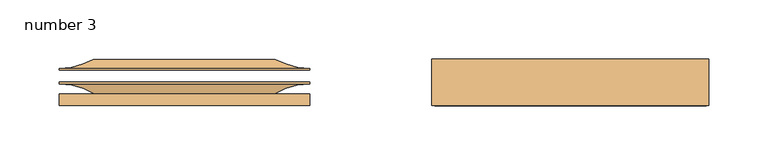
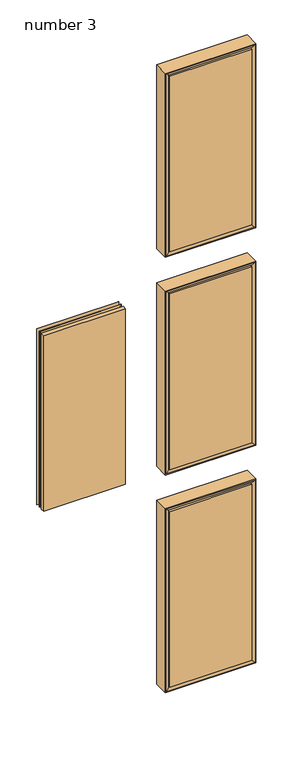
"""IFC4 building model written with IfcOpenShell, lengths in millimetres: door geometry, Door-Interior-Karona-K5660-6_Panel : number 3."""

from ifc_helpers import new_model, si_unit, frame, origin, place, context, project, spatial, polyline, ellipse_curve, source, transform, mapped, element, save
from ifc_brep_helpers import plane_surface, cylinder_surface, revolved_surface, advanced_brep


def number_3_bfdb8d82(model_context):
    return source(origin(), model_context, "Body", "AdvancedBrep", [
        advanced_brep(
        [(268.2748, -54.4576, 1893.8748), (57.1627, -54.4576, 1893.8748), (57.1627, -54.4576, 1414.4752), (268.2748, -54.4576, 1414.4752), (268.2748, -34.7218, 1893.8748), (57.1627, -34.7218, 1893.8748), (57.1627, -36.0454899, 1893.8748), (268.2748, -36.0454899, 1893.8748), (268.2748, -44.5515929, 1893.8748), (57.1627, -44.5515929, 1893.8748), (57.1627, -34.7218, 1414.4752), (268.2748, -34.7218, 1414.4752), (268.2748, -36.0454899, 1414.4752), (57.1627, -36.0454899, 1414.4752), (57.1627, -44.5515929, 1414.4752), (268.2748, -44.5515929, 1414.4752), (87.1686653, -44.5515929, 1863.8688347), (238.2688347, -44.5515929, 1863.8688347), (87.1686653, -44.5515929, 1444.4811653), (238.2688347, -44.5515929, 1444.4811653)],
        [
            (0, 1),
            (1, 2),
            (2, 3),
            (3, 0),
            (4, 5),
            (5, 6),
            (6, 7),
            (7, 4),
            (0, 8),
            (8, 9),
            (9, 1),
            (10, 11),
            (11, 12),
            (12, 13),
            (13, 10),
            (2, 14),
            (14, 15),
            (15, 3),
            (15, 8),
            (11, 4),
            (7, 12),
            (9, 14),
            (5, 10),
            (13, 6),
            (16, 17),
            (17, 7, ellipse_curve(frame((270.2131685, -100.0605261, 1895.8131685), z_axis=(0.7071067811865475, 0.0, -0.7071067811865475), x_axis=(0.7071067811865476, 0.0, 0.7071067811865474)), 90.5724254, 64.0443762)),
            (6, 16, ellipse_curve(frame((55.2243315, -100.0605261, 1895.8131685), z_axis=(-0.7071067811865475, 0.0, -0.7071067811865475), x_axis=(0.7071067811865476, 0.0, -0.7071067811865474)), 90.5724254, 64.0443762)),
            (18, 16),
            (13, 18, ellipse_curve(frame((55.2243315, -100.0605261, 1412.5368315), z_axis=(0.7071067811865475, 0.0, -0.7071067811865475), x_axis=(0.7071067811865474, 0.0, 0.7071067811865476)), 90.5724254, 64.0443762)),
            (19, 18),
            (12, 19, ellipse_curve(frame((270.2131685, -100.0605261, 1412.5368315), z_axis=(0.7071067811865475, 0.0, 0.7071067811865475), x_axis=(-0.7071067811865476, 0.0, 0.7071067811865474)), 90.5724254, 64.0443762)),
            (17, 19),
        ],
        [
            plane_surface(frame((57.1627, -54.4576, 1893.8748), z_axis=(0.0, -1.0, 0.0), x_axis=(0.0, 0.0, -1.0))),
            plane_surface(frame((57.1627, -34.7218, 1893.8748), z_axis=(0.0, 0.0, 1.0), x_axis=(-1.0, 0.0, 0.0))),
            plane_surface(frame((57.1627, -34.7218, 1414.4752), z_axis=(0.0, 0.0, -1.0), x_axis=(1.0, 0.0, 0.0))),
            plane_surface(frame((268.2748, -54.4576, 1893.8748), z_axis=(1.0, 0.0, 0.0), x_axis=(0.0, 0.0, -1.0))),
            plane_surface(frame((57.1627, -34.7218, 1893.8748), z_axis=(-1.0, 0.0, 0.0), x_axis=(0.0, 0.0, -1.0))),
            plane_surface(frame((268.2748, -34.7218, 1893.8748), z_axis=(0.0, 1.0, 0.0), x_axis=(0.0, 0.0, -1.0))),
            revolved_surface(polyline([(334.2575446888527, -100.0605261, 1831.7687923), (-8.820044688852704, -100.0605261, 1831.7687923)]), (279.4, -100.0605261, 1895.8131685), (1.0, 0.0, 0.0)),
            revolved_surface(polyline([(119.2687077, -100.0605261, 1959.8575446888528), (119.2687077, -100.0605261, 1348.4924553111473)]), (55.2243315, -100.0605261, 1905.0), (0.0, 0.0, 1.0)),
            revolved_surface(polyline([(-8.820044688852683, -100.0605261, 1476.5812077), (334.2575446888527, -100.0605261, 1476.5812077)]), (46.0375, -100.0605261, 1412.5368315), (-1.0, 0.0, 0.0)),
            revolved_surface(polyline([(206.1687923, -100.0605261, 1348.4924553111473), (206.1687923, -100.0605261, 1959.8575446888526)]), (270.2131685, -100.0605261, 1403.35), (0.0, 0.0, -1.0)),
            plane_surface(frame((279.4, -44.5515929, 1403.35), z_axis=(0.0, 1.0, 0.0), x_axis=(0.0, 0.0, 1.0))),
        ],
        [
            (0, [[1, 2, 3, 4]]),
            (1, [[5, 6, 7, 8]]),
            (1, [[-1, 9, 10, 11]]),
            (2, [[12, 13, 14, 15]]),
            (2, [[-3, 16, 17, 18]]),
            (3, [[-4, -18, 19, -9]]),
            (3, [[20, -8, 21, -13]]),
            (4, [[-2, -11, 22, -16]]),
            (4, [[23, -15, 24, -6]]),
            (5, [[-5, -20, -12, -23]]),
            (6, [[25, 26, -7, 27]]),
            (7, [[28, -27, -24, 29]]),
            (8, [[30, -29, -14, 31]]),
            (9, [[32, -31, -21, -26]]),
            (10, [[-10, -19, -17, -22], [-25, -28, -30, -32]]),
        ],
    ),
        advanced_brep(
        [(268.2748, -24.6126, 1893.8748), (57.1627, -24.6126, 1893.8748), (57.1627, -24.6126, 1414.4752), (268.2748, -24.6126, 1414.4752), (239.4448579, -15.4432, 1443.3051421), (85.9926421, -15.4432, 1443.3051421), (85.9926421, -15.4432, 1865.0448579), (239.4448579, -15.4432, 1865.0448579), (268.2748, -23.2889101, 1893.8748), (57.1627, -23.2889101, 1893.8748), (57.1627, -23.2889101, 1414.4752), (268.2748, -23.2889101, 1414.4752)],
        [
            (0, 1),
            (1, 2),
            (2, 3),
            (3, 0),
            (4, 5),
            (5, 6),
            (6, 7),
            (7, 4),
            (0, 8),
            (8, 9),
            (9, 1),
            (2, 10),
            (10, 11),
            (11, 3),
            (4, 11, ellipse_curve(frame((270.2131685, 40.7261261, 1412.5368315), z_axis=(0.7071067811865475, 0.0, 0.7071067811865475), x_axis=(-0.7071067811865476, 0.0, 0.7071067811865474)), 90.5724254, 64.0443762)),
            (10, 5, ellipse_curve(frame((55.2243315, 40.7261261, 1412.5368315), z_axis=(-0.7071067811865475, 0.0, 0.7071067811865475), x_axis=(-0.7071067811865476, 0.0, -0.7071067811865474)), 90.5724254, 64.0443762)),
            (7, 8, ellipse_curve(frame((270.2131685, 40.7261261, 1895.8131685), z_axis=(-0.7071067811865475, 0.0, 0.7071067811865475), x_axis=(-0.7071067811865474, 0.0, -0.7071067811865476)), 90.5724254, 64.0443762)),
            (8, 11),
            (6, 9, ellipse_curve(frame((55.2243315, 40.7261261, 1895.8131685), z_axis=(-0.7071067811865475, 0.0, -0.7071067811865475), x_axis=(0.7071067811865476, 0.0, -0.7071067811865474)), 90.5724254, 64.0443762)),
            (10, 9),
        ],
        [
            plane_surface(frame((57.1627, -24.6126, 1893.8748), z_axis=(0.0, -1.0, 0.0), x_axis=(0.0, 0.0, -1.0))),
            plane_surface(frame((268.2748, -15.4432, 1893.8748), z_axis=(0.0, 1.0, 0.0), x_axis=(0.0, 0.0, -1.0))),
            plane_surface(frame((57.1627, -34.7218, 1893.8748), z_axis=(0.0, 0.0, 1.0), x_axis=(-1.0, 0.0, 0.0))),
            plane_surface(frame((57.1627, -34.7218, 1414.4752), z_axis=(0.0, 0.0, -1.0), x_axis=(1.0, 0.0, 0.0))),
            revolved_surface(polyline([(-8.820044688852711, 40.7261261, 1476.5812077), (334.2575446888527, 40.7261261, 1476.5812077)]), (46.0375, 40.7261261, 1412.5368315), (-1.0, 0.0, 0.0)),
            revolved_surface(polyline([(206.1687923, 40.7261261, 1348.4924553111473), (206.1687923, 40.7261261, 1959.8575446888528)]), (270.2131685, 40.7261261, 1403.35), (0.0, 0.0, -1.0)),
            revolved_surface(polyline([(334.2575446888527, 40.7261261, 1831.7687923), (-8.820044688852704, 40.7261261, 1831.7687923)]), (279.4, 40.7261261, 1895.8131685), (1.0, 0.0, 0.0)),
            revolved_surface(polyline([(119.2687077, 40.7261261, 1959.8575446888528), (119.2687077, 40.7261261, 1348.4924553111473)]), (55.2243315, 40.7261261, 1905.0), (0.0, 0.0, 1.0)),
            plane_surface(frame((268.2748, -24.6126, 1893.8748), z_axis=(1.0, 0.0, 0.0), x_axis=(0.0, 0.0, -1.0))),
            plane_surface(frame((57.1627, -15.4432, 1893.8748), z_axis=(-1.0, 0.0, 0.0), x_axis=(0.0, 0.0, -1.0))),
        ],
        [
            (0, [[1, 2, 3, 4]]),
            (1, [[5, 6, 7, 8]]),
            (2, [[-1, 9, 10, 11]]),
            (3, [[-3, 12, 13, 14]]),
            (4, [[15, -13, 16, -5]]),
            (5, [[-15, -8, 17, 18]]),
            (6, [[-17, -7, 19, -10]]),
            (7, [[-19, -6, -16, 20]]),
            (8, [[-4, -14, -18, -9]]),
            (9, [[-2, -11, -20, -12]]),
        ],
    ),
        advanced_brep(
        [(279.4, -15.2908, 1905.0), (268.0746863, -24.6126, 1893.6746863), (57.3628137, -24.6126, 1893.6746863), (46.0375, -15.2908, 1905.0), (57.1627, -46.3324899, 1893.8748), (48.2727, -54.4576, 1902.7648), (48.2727, -54.4576, 1405.5852), (57.1627, -46.3324899, 1414.4752), (268.2748, -46.3324899, 1414.4752), (277.1648, -54.4576, 1405.5852), (277.1648, -54.4576, 1902.7648), (268.2748, -46.3324899, 1893.8748), (46.0375, -54.4576, 1403.35), (46.0375, -15.2908, 1403.35), (279.4, -15.2908, 1403.35), (279.4, -54.4576, 1403.35), (57.1627, -34.7218, 1414.4752), (268.2748, -34.7218, 1414.4752), (47.3075, -24.6126, 1903.73), (47.3075, -34.7218, 1903.73), (47.3075, -34.7218, 1404.62), (47.3075, -24.6126, 1404.62), (278.13, -24.6126, 1404.62), (278.13, -24.6126, 1903.73), (57.3628137, -24.6126, 1414.6753137), (268.0746863, -24.6126, 1414.6753137), (278.13, -34.7218, 1404.62), (279.4, -54.4576, 1905.0), (268.2748, -34.7218, 1893.8748), (278.13, -34.7218, 1903.73), (46.0375, -54.4576, 1905.0), (57.1627, -34.7218, 1893.8748)],
        [
            (0, 1, ellipse_curve(frame((278.3689876, -25.5788135, 1903.9689876), z_axis=(-0.7071067811865475, 0.0, 0.7071067811865475), x_axis=(0.7071067811865476, 0.0, 0.7071067811865474)), 14.6223259, 10.3395458)),
            (1, 2),
            (2, 3, ellipse_curve(frame((47.0685124, -25.5788135, 1903.9689876), z_axis=(0.7071067811865475, 0.0, 0.7071067811865475), x_axis=(0.7071067811865476, 0.0, -0.7071067811865474)), 14.6223259, 10.3395458)),
            (3, 0),
            (4, 5, ellipse_curve(frame((48.2727, -45.531597, 1902.7648), z_axis=(-0.7071067811865475, 0.0, -0.7071067811865475), x_axis=(-0.7071067811865474, 0.0, 0.7071067811865476)), 12.6232745, 8.926003)),
            (5, 6),
            (6, 7, ellipse_curve(frame((48.2727, -45.531597, 1405.5852), z_axis=(-0.7071067811865475, 0.0, 0.7071067811865475), x_axis=(0.7071067811865474, 0.0, 0.7071067811865476)), 12.6232745, 8.926003)),
            (7, 4),
            (8, 9, ellipse_curve(frame((277.1648, -45.531597, 1405.5852), z_axis=(0.7071067811865475, 0.0, 0.7071067811865475), x_axis=(0.7071067811865474, 0.0, -0.7071067811865476)), 12.6232745, 8.926003)),
            (9, 10),
            (10, 11, ellipse_curve(frame((277.1648, -45.531597, 1902.7648), z_axis=(0.7071067811865475, 0.0, -0.7071067811865475), x_axis=(-0.7071067811865474, 0.0, -0.7071067811865476)), 12.6232745, 8.926003)),
            (11, 8),
            (12, 13),
            (13, 14),
            (14, 15),
            (15, 12),
            (16, 7),
            (7, 8),
            (8, 17),
            (17, 16),
            (18, 19),
            (19, 20),
            (20, 21),
            (21, 18),
            (22, 23),
            (23, 18),
            (21, 22),
            (24, 2),
            (1, 25),
            (25, 24),
            (20, 26),
            (26, 22),
            (14, 0),
            (0, 27),
            (27, 15),
            (11, 28),
            (28, 17),
            (26, 29),
            (29, 23),
            (3, 30),
            (30, 27),
            (11, 4),
            (4, 31),
            (31, 28),
            (29, 19),
            (3, 13),
            (12, 30),
            (16, 31),
            (5, 10),
            (9, 6),
            (13, 24, ellipse_curve(frame((47.0685124, -25.5788135, 1404.3810124), z_axis=(0.7071067811865475, 0.0, -0.7071067811865475), x_axis=(-0.7071067811865476, 0.0, -0.7071067811865474)), 14.6223259, 10.3395458)),
            (25, 14, ellipse_curve(frame((278.3689876, -25.5788135, 1404.3810124), z_axis=(-0.7071067811865475, 0.0, -0.7071067811865475), x_axis=(-0.7071067811865476, 0.0, 0.7071067811865474)), 14.6223259, 10.3395458)),
        ],
        [
            cylinder_surface(frame((279.4, -25.5788135, 1903.9689876), z_axis=(1.0, 0.0, 0.0), x_axis=(0.0, 1.0, 0.0)), 10.3395458),
            cylinder_surface(frame((48.2727, -45.531597, 1905.0), z_axis=(0.0, 0.0, 1.0), x_axis=(0.0, 1.0, 0.0)), 8.926003),
            cylinder_surface(frame((277.1648, -45.531597, 1403.35), z_axis=(0.0, 0.0, -1.0), x_axis=(0.0, 1.0, 0.0)), 8.926003),
            plane_surface(frame((46.0375, -15.2908, 1403.35), z_axis=(0.0, 0.0, -1.0), x_axis=(1.0, 0.0, 0.0))),
            plane_surface(frame((57.1627, -46.3324899, 1414.4752), z_axis=(0.0, 0.0, 1.0), x_axis=(1.0, 0.0, 0.0))),
            plane_surface(frame((47.3075, -34.7218, 1903.73), z_axis=(1.0, 0.0, 0.0), x_axis=(0.0, 0.0, -1.0))),
            plane_surface(frame((47.3075, -24.6126, 1903.73), z_axis=(0.0, -1.0, 0.0), x_axis=(0.0, 0.0, -1.0))),
            plane_surface(frame((47.3075, -34.7218, 1404.62), z_axis=(0.0, 0.0, 1.0), x_axis=(1.0, 0.0, 0.0))),
            plane_surface(frame((279.4, -15.2908, 1403.35), z_axis=(1.0, 0.0, 0.0), x_axis=(0.0, 0.0, 1.0))),
            plane_surface(frame((268.2748, -46.3324899, 1414.4752), z_axis=(-1.0, 0.0, 0.0), x_axis=(0.0, 0.0, 1.0))),
            plane_surface(frame((278.13, -34.7218, 1404.62), z_axis=(-1.0, 0.0, 0.0), x_axis=(0.0, 0.0, 1.0))),
            plane_surface(frame((279.4, -15.2908, 1905.0), z_axis=(0.0, 0.0, 1.0), x_axis=(-1.0, 0.0, 0.0))),
            plane_surface(frame((268.2748, -46.3324899, 1893.8748), z_axis=(0.0, 0.0, -1.0), x_axis=(-1.0, 0.0, 0.0))),
            plane_surface(frame((278.13, -34.7218, 1903.73), z_axis=(0.0, 0.0, -1.0), x_axis=(-1.0, 0.0, 0.0))),
            plane_surface(frame((46.0375, -15.2908, 1905.0), z_axis=(-1.0, 0.0, 0.0), x_axis=(0.0, 0.0, -1.0))),
            plane_surface(frame((57.1627, -46.3324899, 1893.8748), z_axis=(1.0, 0.0, 0.0), x_axis=(0.0, 0.0, -1.0))),
            plane_surface(frame((57.1627, -34.7218, 1893.8748), z_axis=(0.0, 1.0, 0.0), x_axis=(0.0, 0.0, -1.0))),
            plane_surface(frame((46.0375, -54.4576, 1905.0), z_axis=(0.0, -1.0, 0.0), x_axis=(0.0, 0.0, -1.0))),
            cylinder_surface(frame((46.0375, -45.531597, 1405.5852), z_axis=(-1.0, 0.0, 0.0), x_axis=(0.0, 1.0, 0.0)), 8.926003),
            cylinder_surface(frame((46.0375, -25.5788135, 1404.3810124), z_axis=(-1.0, 0.0, 0.0), x_axis=(0.0, 1.0, 0.0)), 10.3395458),
            cylinder_surface(frame((278.3689876, -25.5788135, 1403.35), z_axis=(0.0, 0.0, -1.0), x_axis=(0.0, 1.0, 0.0)), 10.3395458),
            cylinder_surface(frame((279.4, -45.531597, 1902.7648), z_axis=(1.0, 0.0, 0.0), x_axis=(0.0, 1.0, 0.0)), 8.926003),
            cylinder_surface(frame((47.0685124, -25.5788135, 1905.0), z_axis=(0.0, 0.0, 1.0), x_axis=(0.0, 1.0, 0.0)), 10.3395458),
        ],
        [
            (0, [[1, 2, 3, 4]]),
            (1, [[5, 6, 7, 8]]),
            (2, [[9, 10, 11, 12]]),
            (3, [[13, 14, 15, 16]]),
            (4, [[17, 18, 19, 20]]),
            (5, [[21, 22, 23, 24]]),
            (6, [[25, 26, -24, 27], [28, -2, 29, 30]]),
            (7, [[-23, 31, 32, -27]]),
            (8, [[-15, 33, 34, 35]]),
            (9, [[-19, -12, 36, 37]]),
            (10, [[-32, 38, 39, -25]]),
            (11, [[-34, -4, 40, 41]]),
            (12, [[-36, 42, 43, 44]]),
            (13, [[-39, 45, -21, -26]]),
            (14, [[-40, 46, -13, 47]]),
            (15, [[-43, -8, -17, 48]]),
            (16, [[-22, -45, -38, -31], [-37, -44, -48, -20]]),
            (17, [[-35, -41, -47, -16], [-6, 49, -10, 50]]),
            (18, [[-7, -50, -9, -18]]),
            (19, [[51, -30, 52, -14]]),
            (20, [[-52, -29, -1, -33]]),
            (21, [[-11, -49, -5, -42]]),
            (22, [[-3, -28, -51, -46]]),
        ],
    ),
        advanced_brep(
        [(268.2748, -54.4576, 1300.1498), (57.1627, -54.4576, 1300.1498), (57.1627, -54.4576, 820.7502), (268.2748, -54.4576, 820.7502), (268.2748, -34.7218, 1300.1498), (57.1627, -34.7218, 1300.1498), (57.1627, -36.0454899, 1300.1498), (268.2748, -36.0454899, 1300.1498), (268.2748, -44.5515929, 1300.1498), (57.1627, -44.5515929, 1300.1498), (57.1627, -34.7218, 820.7502), (268.2748, -34.7218, 820.7502), (268.2748, -36.0454899, 820.7502), (57.1627, -36.0454899, 820.7502), (57.1627, -44.5515929, 820.7502), (268.2748, -44.5515929, 820.7502), (87.1686653, -44.5515929, 1270.1438347), (238.2688347, -44.5515929, 1270.1438347), (87.1686653, -44.5515929, 850.7561653), (238.2688347, -44.5515929, 850.7561653)],
        [
            (0, 1),
            (1, 2),
            (2, 3),
            (3, 0),
            (4, 5),
            (5, 6),
            (6, 7),
            (7, 4),
            (0, 8),
            (8, 9),
            (9, 1),
            (10, 11),
            (11, 12),
            (12, 13),
            (13, 10),
            (2, 14),
            (14, 15),
            (15, 3),
            (15, 8),
            (11, 4),
            (7, 12),
            (9, 14),
            (5, 10),
            (13, 6),
            (16, 17),
            (17, 7, ellipse_curve(frame((270.2131685, -100.0605261, 1302.0881685), z_axis=(0.7071067811865475, 0.0, -0.7071067811865475), x_axis=(0.7071067811865476, 0.0, 0.7071067811865474)), 90.5724254, 64.0443762)),
            (6, 16, ellipse_curve(frame((55.2243315, -100.0605261, 1302.0881685), z_axis=(-0.7071067811865475, 0.0, -0.7071067811865475), x_axis=(0.7071067811865476, 0.0, -0.7071067811865474)), 90.5724254, 64.0443762)),
            (18, 16),
            (13, 18, ellipse_curve(frame((55.2243315, -100.0605261, 818.8118315), z_axis=(0.7071067811865475, 0.0, -0.7071067811865475), x_axis=(0.7071067811865474, 0.0, 0.7071067811865476)), 90.5724254, 64.0443762)),
            (19, 18),
            (12, 19, ellipse_curve(frame((270.2131685, -100.0605261, 818.8118315), z_axis=(0.7071067811865475, 0.0, 0.7071067811865475), x_axis=(-0.7071067811865476, 0.0, 0.7071067811865474)), 90.5724254, 64.0443762)),
            (17, 19),
        ],
        [
            plane_surface(frame((57.1627, -54.4576, 1300.1498), z_axis=(0.0, -1.0, 0.0), x_axis=(0.0, 0.0, -1.0))),
            plane_surface(frame((57.1627, -34.7218, 1300.1498), z_axis=(0.0, 0.0, 1.0), x_axis=(-1.0, 0.0, 0.0))),
            plane_surface(frame((57.1627, -34.7218, 820.7502), z_axis=(0.0, 0.0, -1.0), x_axis=(1.0, 0.0, 0.0))),
            plane_surface(frame((268.2748, -54.4576, 1300.1498), z_axis=(1.0, 0.0, 0.0), x_axis=(0.0, 0.0, -1.0))),
            plane_surface(frame((57.1627, -34.7218, 1300.1498), z_axis=(-1.0, 0.0, 0.0), x_axis=(0.0, 0.0, -1.0))),
            plane_surface(frame((268.2748, -34.7218, 1300.1498), z_axis=(0.0, 1.0, 0.0), x_axis=(0.0, 0.0, -1.0))),
            revolved_surface(polyline([(334.2575446888527, -100.0605261, 1238.0437923), (-8.820044688852704, -100.0605261, 1238.0437923)]), (279.4, -100.0605261, 1302.0881685), (1.0, 0.0, 0.0)),
            revolved_surface(polyline([(119.2687077, -100.0605261, 1366.1325446888527), (119.2687077, -100.0605261, 754.7674553111474)]), (55.2243315, -100.0605261, 1311.275), (0.0, 0.0, 1.0)),
            revolved_surface(polyline([(-8.820044688852683, -100.0605261, 882.8562077), (334.2575446888527, -100.0605261, 882.8562077)]), (46.0375, -100.0605261, 818.8118315), (-1.0, 0.0, 0.0)),
            revolved_surface(polyline([(206.1687923, -100.0605261, 754.7674553111474), (206.1687923, -100.0605261, 1366.1325446888527)]), (270.2131685, -100.0605261, 809.625), (0.0, 0.0, -1.0)),
            plane_surface(frame((279.4, -44.5515929, 809.625), z_axis=(0.0, 1.0, 0.0), x_axis=(0.0, 0.0, 1.0))),
        ],
        [
            (0, [[1, 2, 3, 4]]),
            (1, [[5, 6, 7, 8]]),
            (1, [[-1, 9, 10, 11]]),
            (2, [[12, 13, 14, 15]]),
            (2, [[-3, 16, 17, 18]]),
            (3, [[-4, -18, 19, -9]]),
            (3, [[20, -8, 21, -13]]),
            (4, [[-2, -11, 22, -16]]),
            (4, [[23, -15, 24, -6]]),
            (5, [[-5, -20, -12, -23]]),
            (6, [[25, 26, -7, 27]]),
            (7, [[28, -27, -24, 29]]),
            (8, [[30, -29, -14, 31]]),
            (9, [[32, -31, -21, -26]]),
            (10, [[-10, -19, -17, -22], [-25, -28, -30, -32]]),
        ],
    ),
        advanced_brep(
        [(268.2748, -24.6126, 1300.1498), (57.1627, -24.6126, 1300.1498), (57.1627, -24.6126, 820.7502), (268.2748, -24.6126, 820.7502), (239.4448579, -15.4432, 849.5801421), (85.9926421, -15.4432, 849.5801421), (85.9926421, -15.4432, 1271.3198579), (239.4448579, -15.4432, 1271.3198579), (268.2748, -23.2889101, 1300.1498), (57.1627, -23.2889101, 1300.1498), (57.1627, -23.2889101, 820.7502), (268.2748, -23.2889101, 820.7502)],
        [
            (0, 1),
            (1, 2),
            (2, 3),
            (3, 0),
            (4, 5),
            (5, 6),
            (6, 7),
            (7, 4),
            (0, 8),
            (8, 9),
            (9, 1),
            (2, 10),
            (10, 11),
            (11, 3),
            (4, 11, ellipse_curve(frame((270.2131685, 40.7261261, 818.8118315), z_axis=(0.7071067811865475, 0.0, 0.7071067811865475), x_axis=(-0.7071067811865476, 0.0, 0.7071067811865474)), 90.5724254, 64.0443762)),
            (10, 5, ellipse_curve(frame((55.2243315, 40.7261261, 818.8118315), z_axis=(-0.7071067811865475, 0.0, 0.7071067811865475), x_axis=(-0.7071067811865476, 0.0, -0.7071067811865474)), 90.5724254, 64.0443762)),
            (7, 8, ellipse_curve(frame((270.2131685, 40.7261261, 1302.0881685), z_axis=(-0.7071067811865475, 0.0, 0.7071067811865475), x_axis=(-0.7071067811865474, 0.0, -0.7071067811865476)), 90.5724254, 64.0443762)),
            (8, 11),
            (6, 9, ellipse_curve(frame((55.2243315, 40.7261261, 1302.0881685), z_axis=(-0.7071067811865475, 0.0, -0.7071067811865475), x_axis=(0.7071067811865476, 0.0, -0.7071067811865474)), 90.5724254, 64.0443762)),
            (10, 9),
        ],
        [
            plane_surface(frame((57.1627, -24.6126, 1300.1498), z_axis=(0.0, -1.0, 0.0), x_axis=(0.0, 0.0, -1.0))),
            plane_surface(frame((268.2748, -15.4432, 1300.1498), z_axis=(0.0, 1.0, 0.0), x_axis=(0.0, 0.0, -1.0))),
            plane_surface(frame((57.1627, -34.7218, 1300.1498), z_axis=(0.0, 0.0, 1.0), x_axis=(-1.0, 0.0, 0.0))),
            plane_surface(frame((57.1627, -34.7218, 820.7502), z_axis=(0.0, 0.0, -1.0), x_axis=(1.0, 0.0, 0.0))),
            revolved_surface(polyline([(-8.820044688852711, 40.7261261, 882.8562077), (334.2575446888527, 40.7261261, 882.8562077)]), (46.0375, 40.7261261, 818.8118315), (-1.0, 0.0, 0.0)),
            revolved_surface(polyline([(206.1687923, 40.7261261, 754.7674553111474), (206.1687923, 40.7261261, 1366.1325446888527)]), (270.2131685, 40.7261261, 809.625), (0.0, 0.0, -1.0)),
            revolved_surface(polyline([(334.2575446888527, 40.7261261, 1238.0437923), (-8.820044688852704, 40.7261261, 1238.0437923)]), (279.4, 40.7261261, 1302.0881685), (1.0, 0.0, 0.0)),
            revolved_surface(polyline([(119.2687077, 40.7261261, 1366.1325446888527), (119.2687077, 40.7261261, 754.7674553111474)]), (55.2243315, 40.7261261, 1311.275), (0.0, 0.0, 1.0)),
            plane_surface(frame((268.2748, -24.6126, 1300.1498), z_axis=(1.0, 0.0, 0.0), x_axis=(0.0, 0.0, -1.0))),
            plane_surface(frame((57.1627, -15.4432, 1300.1498), z_axis=(-1.0, 0.0, 0.0), x_axis=(0.0, 0.0, -1.0))),
        ],
        [
            (0, [[1, 2, 3, 4]]),
            (1, [[5, 6, 7, 8]]),
            (2, [[-1, 9, 10, 11]]),
            (3, [[-3, 12, 13, 14]]),
            (4, [[15, -13, 16, -5]]),
            (5, [[-15, -8, 17, 18]]),
            (6, [[-17, -7, 19, -10]]),
            (7, [[-19, -6, -16, 20]]),
            (8, [[-4, -14, -18, -9]]),
            (9, [[-2, -11, -20, -12]]),
        ],
    ),
        advanced_brep(
        [(279.4, -15.2908, 1311.275), (268.0746863, -24.6126, 1299.9496863), (57.3628137, -24.6126, 1299.9496863), (46.0375, -15.2908, 1311.275), (57.1627, -46.3324899, 1300.1498), (48.2727, -54.4576, 1309.0398), (48.2727, -54.4576, 811.8602), (57.1627, -46.3324899, 820.7502), (268.2748, -46.3324899, 820.7502), (277.1648, -54.4576, 811.8602), (277.1648, -54.4576, 1309.0398), (268.2748, -46.3324899, 1300.1498), (46.0375, -54.4576, 809.625), (46.0375, -15.2908, 809.625), (279.4, -15.2908, 809.625), (279.4, -54.4576, 809.625), (57.1627, -34.7218, 820.7502), (268.2748, -34.7218, 820.7502), (47.3075, -24.6126, 1310.005), (47.3075, -34.7218, 1310.005), (47.3075, -34.7218, 810.895), (47.3075, -24.6126, 810.895), (278.13, -24.6126, 810.895), (278.13, -24.6126, 1310.005), (57.3628137, -24.6126, 820.9503137), (268.0746863, -24.6126, 820.9503137), (278.13, -34.7218, 810.895), (279.4, -54.4576, 1311.275), (268.2748, -34.7218, 1300.1498), (278.13, -34.7218, 1310.005), (46.0375, -54.4576, 1311.275), (57.1627, -34.7218, 1300.1498)],
        [
            (0, 1, ellipse_curve(frame((278.3689876, -25.5788135, 1310.2439876), z_axis=(-0.7071067811865475, 0.0, 0.7071067811865475), x_axis=(0.7071067811865476, 0.0, 0.7071067811865474)), 14.6223259, 10.3395458)),
            (1, 2),
            (2, 3, ellipse_curve(frame((47.0685124, -25.5788135, 1310.2439876), z_axis=(0.7071067811865475, 0.0, 0.7071067811865475), x_axis=(0.7071067811865476, 0.0, -0.7071067811865474)), 14.6223259, 10.3395458)),
            (3, 0),
            (4, 5, ellipse_curve(frame((48.2727, -45.531597, 1309.0398), z_axis=(-0.7071067811865475, 0.0, -0.7071067811865475), x_axis=(-0.7071067811865474, 0.0, 0.7071067811865476)), 12.6232745, 8.926003)),
            (5, 6),
            (6, 7, ellipse_curve(frame((48.2727, -45.531597, 811.8602), z_axis=(-0.7071067811865475, 0.0, 0.7071067811865475), x_axis=(0.7071067811865474, 0.0, 0.7071067811865476)), 12.6232745, 8.926003)),
            (7, 4),
            (8, 9, ellipse_curve(frame((277.1648, -45.531597, 811.8602), z_axis=(0.7071067811865475, 0.0, 0.7071067811865475), x_axis=(0.7071067811865474, 0.0, -0.7071067811865476)), 12.6232745, 8.926003)),
            (9, 10),
            (10, 11, ellipse_curve(frame((277.1648, -45.531597, 1309.0398), z_axis=(0.7071067811865475, 0.0, -0.7071067811865475), x_axis=(-0.7071067811865474, 0.0, -0.7071067811865476)), 12.6232745, 8.926003)),
            (11, 8),
            (12, 13),
            (13, 14),
            (14, 15),
            (15, 12),
            (16, 7),
            (7, 8),
            (8, 17),
            (17, 16),
            (18, 19),
            (19, 20),
            (20, 21),
            (21, 18),
            (22, 23),
            (23, 18),
            (21, 22),
            (24, 2),
            (1, 25),
            (25, 24),
            (13, 24, ellipse_curve(frame((47.0685124, -25.5788135, 810.6560124), z_axis=(0.7071067811865475, 0.0, -0.7071067811865475), x_axis=(-0.7071067811865476, 0.0, -0.7071067811865474)), 14.6223259, 10.3395458)),
            (25, 14, ellipse_curve(frame((278.3689876, -25.5788135, 810.6560124), z_axis=(-0.7071067811865475, 0.0, -0.7071067811865475), x_axis=(-0.7071067811865476, 0.0, 0.7071067811865474)), 14.6223259, 10.3395458)),
            (20, 26),
            (26, 22),
            (14, 0),
            (0, 27),
            (27, 15),
            (11, 28),
            (28, 17),
            (26, 29),
            (29, 23),
            (3, 30),
            (30, 27),
            (11, 4),
            (4, 31),
            (31, 28),
            (29, 19),
            (3, 13),
            (12, 30),
            (16, 31),
            (5, 10),
            (9, 6),
        ],
        [
            cylinder_surface(frame((279.4, -25.5788135, 1310.2439876), z_axis=(1.0, 0.0, 0.0), x_axis=(0.0, 1.0, 0.0)), 10.3395458),
            cylinder_surface(frame((48.2727, -45.531597, 1311.275), z_axis=(0.0, 0.0, 1.0), x_axis=(0.0, 1.0, 0.0)), 8.926003),
            cylinder_surface(frame((277.1648, -45.531597, 809.625), z_axis=(0.0, 0.0, -1.0), x_axis=(0.0, 1.0, 0.0)), 8.926003),
            plane_surface(frame((46.0375, -15.2908, 809.625), z_axis=(0.0, 0.0, -1.0), x_axis=(1.0, 0.0, 0.0))),
            plane_surface(frame((57.1627, -46.3324899, 820.7502), z_axis=(0.0, 0.0, 1.0), x_axis=(1.0, 0.0, 0.0))),
            plane_surface(frame((47.3075, -34.7218, 1310.005), z_axis=(1.0, 0.0, 0.0), x_axis=(0.0, 0.0, -1.0))),
            plane_surface(frame((47.3075, -24.6126, 1310.005), z_axis=(0.0, -1.0, 0.0), x_axis=(0.0, 0.0, -1.0))),
            cylinder_surface(frame((46.0375, -25.5788135, 810.6560124), z_axis=(-1.0, 0.0, 0.0), x_axis=(0.0, 1.0, 0.0)), 10.3395458),
            plane_surface(frame((47.3075, -34.7218, 810.895), z_axis=(0.0, 0.0, 1.0), x_axis=(1.0, 0.0, 0.0))),
            plane_surface(frame((279.4, -15.2908, 809.625), z_axis=(1.0, 0.0, 0.0), x_axis=(0.0, 0.0, 1.0))),
            plane_surface(frame((268.2748, -46.3324899, 820.7502), z_axis=(-1.0, 0.0, 0.0), x_axis=(0.0, 0.0, 1.0))),
            plane_surface(frame((278.13, -34.7218, 810.895), z_axis=(-1.0, 0.0, 0.0), x_axis=(0.0, 0.0, 1.0))),
            plane_surface(frame((279.4, -15.2908, 1311.275), z_axis=(0.0, 0.0, 1.0), x_axis=(-1.0, 0.0, 0.0))),
            plane_surface(frame((268.2748, -46.3324899, 1300.1498), z_axis=(0.0, 0.0, -1.0), x_axis=(-1.0, 0.0, 0.0))),
            plane_surface(frame((278.13, -34.7218, 1310.005), z_axis=(0.0, 0.0, -1.0), x_axis=(-1.0, 0.0, 0.0))),
            plane_surface(frame((46.0375, -15.2908, 1311.275), z_axis=(-1.0, 0.0, 0.0), x_axis=(0.0, 0.0, -1.0))),
            plane_surface(frame((57.1627, -46.3324899, 1300.1498), z_axis=(1.0, 0.0, 0.0), x_axis=(0.0, 0.0, -1.0))),
            plane_surface(frame((57.1627, -34.7218, 1300.1498), z_axis=(0.0, 1.0, 0.0), x_axis=(0.0, 0.0, -1.0))),
            plane_surface(frame((46.0375, -54.4576, 1311.275), z_axis=(0.0, -1.0, 0.0), x_axis=(0.0, 0.0, -1.0))),
            cylinder_surface(frame((46.0375, -45.531597, 811.8602), z_axis=(-1.0, 0.0, 0.0), x_axis=(0.0, 1.0, 0.0)), 8.926003),
            cylinder_surface(frame((278.3689876, -25.5788135, 809.625), z_axis=(0.0, 0.0, -1.0), x_axis=(0.0, 1.0, 0.0)), 10.3395458),
            cylinder_surface(frame((279.4, -45.531597, 1309.0398), z_axis=(1.0, 0.0, 0.0), x_axis=(0.0, 1.0, 0.0)), 8.926003),
            cylinder_surface(frame((47.0685124, -25.5788135, 1311.275), z_axis=(0.0, 0.0, 1.0), x_axis=(0.0, 1.0, 0.0)), 10.3395458),
        ],
        [
            (0, [[1, 2, 3, 4]]),
            (1, [[5, 6, 7, 8]]),
            (2, [[9, 10, 11, 12]]),
            (3, [[13, 14, 15, 16]]),
            (4, [[17, 18, 19, 20]]),
            (5, [[21, 22, 23, 24]]),
            (6, [[25, 26, -24, 27], [28, -2, 29, 30]]),
            (7, [[31, -30, 32, -14]]),
            (8, [[-23, 33, 34, -27]]),
            (9, [[-15, 35, 36, 37]]),
            (10, [[-19, -12, 38, 39]]),
            (11, [[-34, 40, 41, -25]]),
            (12, [[-36, -4, 42, 43]]),
            (13, [[-38, 44, 45, 46]]),
            (14, [[-41, 47, -21, -26]]),
            (15, [[-42, 48, -13, 49]]),
            (16, [[-45, -8, -17, 50]]),
            (17, [[-22, -47, -40, -33], [-39, -46, -50, -20]]),
            (18, [[-37, -43, -49, -16], [-6, 51, -10, 52]]),
            (19, [[-7, -52, -9, -18]]),
            (20, [[-32, -29, -1, -35]]),
            (21, [[-11, -51, -5, -44]]),
            (22, [[-3, -28, -31, -48]]),
        ],
    ),
        advanced_brep(
        [(268.2748, -54.4576, 706.4248), (57.1627, -54.4576, 706.4248), (57.1627, -54.4576, 227.0252), (268.2748, -54.4576, 227.0252), (268.2748, -34.7218, 706.4248), (57.1627, -34.7218, 706.4248), (57.1627, -36.0454899, 706.4248), (268.2748, -36.0454899, 706.4248), (268.2748, -44.5515929, 706.4248), (57.1627, -44.5515929, 706.4248), (57.1627, -34.7218, 227.0252), (268.2748, -34.7218, 227.0252), (268.2748, -36.0454899, 227.0252), (57.1627, -36.0454899, 227.0252), (57.1627, -44.5515929, 227.0252), (268.2748, -44.5515929, 227.0252), (87.1686653, -44.5515929, 676.4188347), (238.2688347, -44.5515929, 676.4188347), (87.1686653, -44.5515929, 257.0311653), (238.2688347, -44.5515929, 257.0311653)],
        [
            (0, 1),
            (1, 2),
            (2, 3),
            (3, 0),
            (4, 5),
            (5, 6),
            (6, 7),
            (7, 4),
            (0, 8),
            (8, 9),
            (9, 1),
            (10, 11),
            (11, 12),
            (12, 13),
            (13, 10),
            (2, 14),
            (14, 15),
            (15, 3),
            (15, 8),
            (11, 4),
            (7, 12),
            (9, 14),
            (5, 10),
            (13, 6),
            (16, 17),
            (17, 7, ellipse_curve(frame((270.2131685, -100.0605261, 708.3631685), z_axis=(0.7071067811865475, 0.0, -0.7071067811865475), x_axis=(0.7071067811865476, 0.0, 0.7071067811865474)), 90.5724254, 64.0443762)),
            (6, 16, ellipse_curve(frame((55.2243315, -100.0605261, 708.3631685), z_axis=(-0.7071067811865475, 0.0, -0.7071067811865475), x_axis=(0.7071067811865476, 0.0, -0.7071067811865474)), 90.5724254, 64.0443762)),
            (18, 16),
            (13, 18, ellipse_curve(frame((55.2243315, -100.0605261, 225.0868315), z_axis=(0.7071067811865475, 0.0, -0.7071067811865475), x_axis=(0.7071067811865474, 0.0, 0.7071067811865476)), 90.5724254, 64.0443762)),
            (19, 18),
            (12, 19, ellipse_curve(frame((270.2131685, -100.0605261, 225.0868315), z_axis=(0.7071067811865475, 0.0, 0.7071067811865475), x_axis=(-0.7071067811865476, 0.0, 0.7071067811865474)), 90.5724254, 64.0443762)),
            (17, 19),
        ],
        [
            plane_surface(frame((57.1627, -54.4576, 706.4248), z_axis=(0.0, -1.0, 0.0), x_axis=(0.0, 0.0, -1.0))),
            plane_surface(frame((57.1627, -34.7218, 706.4248), z_axis=(0.0, 0.0, 1.0), x_axis=(-1.0, 0.0, 0.0))),
            plane_surface(frame((57.1627, -34.7218, 227.0252), z_axis=(0.0, 0.0, -1.0), x_axis=(1.0, 0.0, 0.0))),
            plane_surface(frame((268.2748, -54.4576, 706.4248), z_axis=(1.0, 0.0, 0.0), x_axis=(0.0, 0.0, -1.0))),
            plane_surface(frame((57.1627, -34.7218, 706.4248), z_axis=(-1.0, 0.0, 0.0), x_axis=(0.0, 0.0, -1.0))),
            plane_surface(frame((268.2748, -34.7218, 706.4248), z_axis=(0.0, 1.0, 0.0), x_axis=(0.0, 0.0, -1.0))),
            revolved_surface(polyline([(334.2575446888527, -100.0605261, 644.3187923), (-8.820044688852704, -100.0605261, 644.3187923)]), (279.4, -100.0605261, 708.3631685), (1.0, 0.0, 0.0)),
            revolved_surface(polyline([(119.2687077, -100.0605261, 772.4075446888527), (119.2687077, -100.0605261, 161.04245531114725)]), (55.2243315, -100.0605261, 717.55), (0.0, 0.0, 1.0)),
            revolved_surface(polyline([(-8.820044688852683, -100.0605261, 289.1312077), (334.2575446888527, -100.0605261, 289.1312077)]), (46.0375, -100.0605261, 225.0868315), (-1.0, 0.0, 0.0)),
            revolved_surface(polyline([(206.1687923, -100.0605261, 161.0424553111473), (206.1687923, -100.0605261, 772.4075446888527)]), (270.2131685, -100.0605261, 215.9), (0.0, 0.0, -1.0)),
            plane_surface(frame((279.4, -44.5515929, 215.9), z_axis=(0.0, 1.0, 0.0), x_axis=(0.0, 0.0, 1.0))),
        ],
        [
            (0, [[1, 2, 3, 4]]),
            (1, [[5, 6, 7, 8]]),
            (1, [[-1, 9, 10, 11]]),
            (2, [[12, 13, 14, 15]]),
            (2, [[-3, 16, 17, 18]]),
            (3, [[-4, -18, 19, -9]]),
            (3, [[20, -8, 21, -13]]),
            (4, [[-2, -11, 22, -16]]),
            (4, [[23, -15, 24, -6]]),
            (5, [[-5, -20, -12, -23]]),
            (6, [[25, 26, -7, 27]]),
            (7, [[28, -27, -24, 29]]),
            (8, [[30, -29, -14, 31]]),
            (9, [[32, -31, -21, -26]]),
            (10, [[-10, -19, -17, -22], [-25, -28, -30, -32]]),
        ],
    ),
        advanced_brep(
        [(268.2748, -24.6126, 706.4248), (57.1627, -24.6126, 706.4248), (57.1627, -24.6126, 227.0252), (268.2748, -24.6126, 227.0252), (239.4448579, -15.4432, 255.8551421), (85.9926421, -15.4432, 255.8551421), (85.9926421, -15.4432, 677.5948579), (239.4448579, -15.4432, 677.5948579), (268.2748, -23.2889101, 706.4248), (57.1627, -23.2889101, 706.4248), (57.1627, -23.2889101, 227.0252), (268.2748, -23.2889101, 227.0252)],
        [
            (0, 1),
            (1, 2),
            (2, 3),
            (3, 0),
            (4, 5),
            (5, 6),
            (6, 7),
            (7, 4),
            (0, 8),
            (8, 9),
            (9, 1),
            (2, 10),
            (10, 11),
            (11, 3),
            (4, 11, ellipse_curve(frame((270.2131685, 40.7261261, 225.0868315), z_axis=(0.7071067811865475, 0.0, 0.7071067811865475), x_axis=(-0.7071067811865476, 0.0, 0.7071067811865474)), 90.5724254, 64.0443762)),
            (10, 5, ellipse_curve(frame((55.2243315, 40.7261261, 225.0868315), z_axis=(-0.7071067811865475, 0.0, 0.7071067811865475), x_axis=(-0.7071067811865476, 0.0, -0.7071067811865474)), 90.5724254, 64.0443762)),
            (7, 8, ellipse_curve(frame((270.2131685, 40.7261261, 708.3631685), z_axis=(-0.7071067811865475, 0.0, 0.7071067811865475), x_axis=(-0.7071067811865474, 0.0, -0.7071067811865476)), 90.5724254, 64.0443762)),
            (8, 11),
            (6, 9, ellipse_curve(frame((55.2243315, 40.7261261, 708.3631685), z_axis=(-0.7071067811865475, 0.0, -0.7071067811865475), x_axis=(0.7071067811865476, 0.0, -0.7071067811865474)), 90.5724254, 64.0443762)),
            (10, 9),
        ],
        [
            plane_surface(frame((57.1627, -24.6126, 706.4248), z_axis=(0.0, -1.0, 0.0), x_axis=(0.0, 0.0, -1.0))),
            plane_surface(frame((268.2748, -15.4432, 706.4248), z_axis=(0.0, 1.0, 0.0), x_axis=(0.0, 0.0, -1.0))),
            plane_surface(frame((57.1627, -34.7218, 706.4248), z_axis=(0.0, 0.0, 1.0), x_axis=(-1.0, 0.0, 0.0))),
            plane_surface(frame((57.1627, -34.7218, 227.0252), z_axis=(0.0, 0.0, -1.0), x_axis=(1.0, 0.0, 0.0))),
            revolved_surface(polyline([(-8.820044688852711, 40.7261261, 289.1312077), (334.2575446888527, 40.7261261, 289.1312077)]), (46.0375, 40.7261261, 225.0868315), (-1.0, 0.0, 0.0)),
            revolved_surface(polyline([(206.1687923, 40.7261261, 161.0424553111473), (206.1687923, 40.7261261, 772.4075446888527)]), (270.2131685, 40.7261261, 215.9), (0.0, 0.0, -1.0)),
            revolved_surface(polyline([(334.2575446888527, 40.7261261, 644.3187923), (-8.820044688852704, 40.7261261, 644.3187923)]), (279.4, 40.7261261, 708.3631685), (1.0, 0.0, 0.0)),
            revolved_surface(polyline([(119.2687077, 40.7261261, 772.4075446888527), (119.2687077, 40.7261261, 161.04245531114736)]), (55.2243315, 40.7261261, 717.55), (0.0, 0.0, 1.0)),
            plane_surface(frame((268.2748, -24.6126, 706.4248), z_axis=(1.0, 0.0, 0.0), x_axis=(0.0, 0.0, -1.0))),
            plane_surface(frame((57.1627, -15.4432, 706.4248), z_axis=(-1.0, 0.0, 0.0), x_axis=(0.0, 0.0, -1.0))),
        ],
        [
            (0, [[1, 2, 3, 4]]),
            (1, [[5, 6, 7, 8]]),
            (2, [[-1, 9, 10, 11]]),
            (3, [[-3, 12, 13, 14]]),
            (4, [[15, -13, 16, -5]]),
            (5, [[-15, -8, 17, 18]]),
            (6, [[-17, -7, 19, -10]]),
            (7, [[-19, -6, -16, 20]]),
            (8, [[-4, -14, -18, -9]]),
            (9, [[-2, -11, -20, -12]]),
        ],
    ),
        advanced_brep(
        [(279.4, -15.2908, 717.55), (268.0746863, -24.6126, 706.2246863), (57.3628137, -24.6126, 706.2246863), (46.0375, -15.2908, 717.55), (57.1627, -46.3324899, 706.4248), (48.2727, -54.4576, 715.3148), (48.2727, -54.4576, 218.1352), (57.1627, -46.3324899, 227.0252), (268.2748, -46.3324899, 227.0252), (277.1648, -54.4576, 218.1352), (277.1648, -54.4576, 715.3148), (268.2748, -46.3324899, 706.4248), (46.0375, -54.4576, 215.9), (46.0375, -15.2908, 215.9), (279.4, -15.2908, 215.9), (279.4, -54.4576, 215.9), (57.1627, -34.7218, 227.0252), (268.2748, -34.7218, 227.0252), (47.3075, -24.6126, 716.28), (47.3075, -34.7218, 716.28), (47.3075, -34.7218, 217.17), (47.3075, -24.6126, 217.17), (278.13, -24.6126, 217.17), (278.13, -24.6126, 716.28), (57.3628137, -24.6126, 227.2253137), (268.0746863, -24.6126, 227.2253137), (278.13, -34.7218, 217.17), (279.4, -54.4576, 717.55), (268.2748, -34.7218, 706.4248), (278.13, -34.7218, 716.28), (46.0375, -54.4576, 717.55), (57.1627, -34.7218, 706.4248)],
        [
            (0, 1, ellipse_curve(frame((278.3689876, -25.5788135, 716.5189876), z_axis=(-0.7071067811865475, 0.0, 0.7071067811865475), x_axis=(0.7071067811865476, 0.0, 0.7071067811865474)), 14.6223259, 10.3395458)),
            (1, 2),
            (2, 3, ellipse_curve(frame((47.0685124, -25.5788135, 716.5189876), z_axis=(0.7071067811865475, 0.0, 0.7071067811865475), x_axis=(0.7071067811865476, 0.0, -0.7071067811865474)), 14.6223259, 10.3395458)),
            (3, 0),
            (4, 5, ellipse_curve(frame((48.2727, -45.531597, 715.3148), z_axis=(-0.7071067811865475, 0.0, -0.7071067811865475), x_axis=(-0.7071067811865474, 0.0, 0.7071067811865476)), 12.6232745, 8.926003)),
            (5, 6),
            (6, 7, ellipse_curve(frame((48.2727, -45.531597, 218.1352), z_axis=(-0.7071067811865475, 0.0, 0.7071067811865475), x_axis=(0.7071067811865474, 0.0, 0.7071067811865476)), 12.6232745, 8.926003)),
            (7, 4),
            (8, 9, ellipse_curve(frame((277.1648, -45.531597, 218.1352), z_axis=(0.7071067811865475, 0.0, 0.7071067811865475), x_axis=(0.7071067811865474, 0.0, -0.7071067811865476)), 12.6232745, 8.926003)),
            (9, 10),
            (10, 11, ellipse_curve(frame((277.1648, -45.531597, 715.3148), z_axis=(0.7071067811865475, 0.0, -0.7071067811865475), x_axis=(-0.7071067811865474, 0.0, -0.7071067811865476)), 12.6232745, 8.926003)),
            (11, 8),
            (12, 13),
            (13, 14),
            (14, 15),
            (15, 12),
            (16, 7),
            (7, 8),
            (8, 17),
            (17, 16),
            (18, 19),
            (19, 20),
            (20, 21),
            (21, 18),
            (22, 23),
            (23, 18),
            (21, 22),
            (24, 2),
            (1, 25),
            (25, 24),
            (13, 24, ellipse_curve(frame((47.0685124, -25.5788135, 216.9310124), z_axis=(0.7071067811865475, 0.0, -0.7071067811865475), x_axis=(-0.7071067811865476, 0.0, -0.7071067811865474)), 14.6223259, 10.3395458)),
            (25, 14, ellipse_curve(frame((278.3689876, -25.5788135, 216.9310124), z_axis=(-0.7071067811865475, 0.0, -0.7071067811865475), x_axis=(-0.7071067811865476, 0.0, 0.7071067811865474)), 14.6223259, 10.3395458)),
            (20, 26),
            (26, 22),
            (14, 0),
            (0, 27),
            (27, 15),
            (11, 28),
            (28, 17),
            (26, 29),
            (29, 23),
            (3, 30),
            (30, 27),
            (11, 4),
            (4, 31),
            (31, 28),
            (29, 19),
            (3, 13),
            (12, 30),
            (16, 31),
            (5, 10),
            (9, 6),
        ],
        [
            cylinder_surface(frame((279.4, -25.5788135, 716.5189876), z_axis=(1.0, 0.0, 0.0), x_axis=(0.0, 1.0, 0.0)), 10.3395458),
            cylinder_surface(frame((48.2727, -45.531597, 717.55), z_axis=(0.0, 0.0, 1.0), x_axis=(0.0, 1.0, 0.0)), 8.926003),
            cylinder_surface(frame((277.1648, -45.531597, 215.9), z_axis=(0.0, 0.0, -1.0), x_axis=(0.0, 1.0, 0.0)), 8.926003),
            plane_surface(frame((46.0375, -15.2908, 215.9), z_axis=(0.0, 0.0, -1.0), x_axis=(1.0, 0.0, 0.0))),
            plane_surface(frame((57.1627, -46.3324899, 227.0252), z_axis=(0.0, 0.0, 1.0), x_axis=(1.0, 0.0, 0.0))),
            plane_surface(frame((47.3075, -34.7218, 716.28), z_axis=(1.0, 0.0, 0.0), x_axis=(0.0, 0.0, -1.0))),
            plane_surface(frame((47.3075, -24.6126, 716.28), z_axis=(0.0, -1.0, 0.0), x_axis=(0.0, 0.0, -1.0))),
            cylinder_surface(frame((46.0375, -25.5788135, 216.9310124), z_axis=(-1.0, 0.0, 0.0), x_axis=(0.0, 1.0, 0.0)), 10.3395458),
            plane_surface(frame((47.3075, -34.7218, 217.17), z_axis=(0.0, 0.0, 1.0), x_axis=(1.0, 0.0, 0.0))),
            plane_surface(frame((279.4, -15.2908, 215.9), z_axis=(1.0, 0.0, 0.0), x_axis=(0.0, 0.0, 1.0))),
            plane_surface(frame((268.2748, -46.3324899, 227.0252), z_axis=(-1.0, 0.0, 0.0), x_axis=(0.0, 0.0, 1.0))),
            plane_surface(frame((278.13, -34.7218, 217.17), z_axis=(-1.0, 0.0, 0.0), x_axis=(0.0, 0.0, 1.0))),
            plane_surface(frame((279.4, -15.2908, 717.55), z_axis=(0.0, 0.0, 1.0), x_axis=(-1.0, 0.0, 0.0))),
            plane_surface(frame((268.2748, -46.3324899, 706.4248), z_axis=(0.0, 0.0, -1.0), x_axis=(-1.0, 0.0, 0.0))),
            plane_surface(frame((278.13, -34.7218, 716.28), z_axis=(0.0, 0.0, -1.0), x_axis=(-1.0, 0.0, 0.0))),
            plane_surface(frame((46.0375, -15.2908, 717.55), z_axis=(-1.0, 0.0, 0.0), x_axis=(0.0, 0.0, -1.0))),
            plane_surface(frame((57.1627, -46.3324899, 706.4248), z_axis=(1.0, 0.0, 0.0), x_axis=(0.0, 0.0, -1.0))),
            plane_surface(frame((57.1627, -34.7218, 706.4248), z_axis=(0.0, 1.0, 0.0), x_axis=(0.0, 0.0, -1.0))),
            plane_surface(frame((46.0375, -54.4576, 717.55), z_axis=(0.0, -1.0, 0.0), x_axis=(0.0, 0.0, -1.0))),
            cylinder_surface(frame((46.0375, -45.531597, 218.1352), z_axis=(-1.0, 0.0, 0.0), x_axis=(0.0, 1.0, 0.0)), 8.926003),
            cylinder_surface(frame((278.3689876, -25.5788135, 215.9), z_axis=(0.0, 0.0, -1.0), x_axis=(0.0, 1.0, 0.0)), 10.3395458),
            cylinder_surface(frame((279.4, -45.531597, 715.3148), z_axis=(1.0, 0.0, 0.0), x_axis=(0.0, 1.0, 0.0)), 8.926003),
            cylinder_surface(frame((47.0685124, -25.5788135, 717.55), z_axis=(0.0, 0.0, 1.0), x_axis=(0.0, 1.0, 0.0)), 10.3395458),
        ],
        [
            (0, [[1, 2, 3, 4]]),
            (1, [[5, 6, 7, 8]]),
            (2, [[9, 10, 11, 12]]),
            (3, [[13, 14, 15, 16]]),
            (4, [[17, 18, 19, 20]]),
            (5, [[21, 22, 23, 24]]),
            (6, [[25, 26, -24, 27], [28, -2, 29, 30]]),
            (7, [[31, -30, 32, -14]]),
            (8, [[-23, 33, 34, -27]]),
            (9, [[-15, 35, 36, 37]]),
            (10, [[-19, -12, 38, 39]]),
            (11, [[-34, 40, 41, -25]]),
            (12, [[-36, -4, 42, 43]]),
            (13, [[-38, 44, 45, 46]]),
            (14, [[-41, 47, -21, -26]]),
            (15, [[-42, 48, -13, 49]]),
            (16, [[-45, -8, -17, 50]]),
            (17, [[-22, -47, -40, -33], [-39, -46, -50, -20]]),
            (18, [[-37, -43, -49, -16], [-6, 51, -10, 52]]),
            (19, [[-7, -52, -9, -18]]),
            (20, [[-32, -29, -1, -35]]),
            (21, [[-11, -51, -5, -44]]),
            (22, [[-3, -28, -31, -48]]),
        ],
    ),
        advanced_brep(
        [(-268.2748, -54.4576, 1300.1498), (-268.2748, -54.4576, 820.7502), (-57.1627, -54.4576, 820.7502), (-57.1627, -54.4576, 1300.1498), (-268.2748, -34.7218, 1300.1498), (-268.2748, -36.0454899, 1300.1498), (-57.1627, -36.0454899, 1300.1498), (-57.1627, -34.7218, 1300.1498), (-57.1627, -44.5515929, 1300.1498), (-268.2748, -44.5515929, 1300.1498), (-57.1627, -34.7218, 820.7502), (-57.1627, -36.0454899, 820.7502), (-268.2748, -36.0454899, 820.7502), (-268.2748, -34.7218, 820.7502), (-268.2748, -44.5515929, 820.7502), (-57.1627, -44.5515929, 820.7502), (-87.1686653, -44.5515929, 1270.1438347), (-238.2688347, -44.5515929, 1270.1438347), (-87.1686653, -44.5515929, 850.7561653), (-238.2688347, -44.5515929, 850.7561653)],
        [
            (0, 1),
            (1, 2),
            (2, 3),
            (3, 0),
            (4, 5),
            (5, 6),
            (6, 7),
            (7, 4),
            (3, 8),
            (8, 9),
            (9, 0),
            (10, 11),
            (11, 12),
            (12, 13),
            (13, 10),
            (1, 14),
            (14, 15),
            (15, 2),
            (9, 14),
            (12, 5),
            (4, 13),
            (6, 11),
            (10, 7),
            (15, 8),
            (16, 6, ellipse_curve(frame((-55.2243315, -100.0605261, 1302.0881685), z_axis=(0.7071067811865475, 0.0, -0.7071067811865475), x_axis=(-0.7071067811865476, 0.0, -0.7071067811865474)), 90.5724254, 64.0443762)),
            (5, 17, ellipse_curve(frame((-270.2131685, -100.0605261, 1302.0881685), z_axis=(-0.7071067811865475, 0.0, -0.7071067811865475), x_axis=(-0.7071067811865476, 0.0, 0.7071067811865474)), 90.5724254, 64.0443762)),
            (17, 16),
            (18, 11, ellipse_curve(frame((-55.2243315, -100.0605261, 818.8118315), z_axis=(-0.7071067811865475, 0.0, -0.7071067811865475), x_axis=(-0.7071067811865474, 0.0, 0.7071067811865476)), 90.5724254, 64.0443762)),
            (16, 18),
            (19, 12, ellipse_curve(frame((-270.2131685, -100.0605261, 818.8118315), z_axis=(-0.7071067811865475, 0.0, 0.7071067811865475), x_axis=(0.7071067811865476, 0.0, 0.7071067811865474)), 90.5724254, 64.0443762)),
            (18, 19),
            (19, 17),
        ],
        [
            plane_surface(frame((-57.1627, -54.4576, 1300.1498), z_axis=(0.0, -1.0, 0.0), x_axis=(0.0, 0.0, -1.0))),
            plane_surface(frame((-57.1627, -34.7218, 1300.1498), z_axis=(0.0, 0.0, 1.0), x_axis=(1.0, 0.0, 0.0))),
            plane_surface(frame((-57.1627, -34.7218, 820.7502), z_axis=(0.0, 0.0, -1.0), x_axis=(-1.0, 0.0, 0.0))),
            plane_surface(frame((-268.2748, -54.4576, 1300.1498), z_axis=(-1.0, 0.0, 0.0), x_axis=(0.0, 0.0, -1.0))),
            plane_surface(frame((-57.1627, -34.7218, 1300.1498), z_axis=(1.0, 0.0, 0.0), x_axis=(0.0, 0.0, -1.0))),
            plane_surface(frame((-268.2748, -34.7218, 1300.1498), z_axis=(0.0, 1.0, 0.0), x_axis=(0.0, 0.0, -1.0))),
            revolved_surface(polyline([(-334.2575446888527, -100.0605261, 1238.0437923), (8.820044688852704, -100.0605261, 1238.0437923)]), (-279.4, -100.0605261, 1302.0881685), (-1.0, 0.0, 0.0)),
            revolved_surface(polyline([(-119.2687077, -100.0605261, 1366.1325446888527), (-119.2687077, -100.0605261, 754.7674553111474)]), (-55.2243315, -100.0605261, 1311.275), (0.0, 0.0, 1.0)),
            revolved_surface(polyline([(8.820044688852683, -100.0605261, 882.8562077), (-334.2575446888527, -100.0605261, 882.8562077)]), (-46.0375, -100.0605261, 818.8118315), (1.0, 0.0, 0.0)),
            revolved_surface(polyline([(-206.1687923, -100.0605261, 754.7674553111474), (-206.1687923, -100.0605261, 1366.1325446888527)]), (-270.2131685, -100.0605261, 809.625), (0.0, 0.0, -1.0)),
            plane_surface(frame((-279.4, -44.5515929, 809.625), z_axis=(0.0, 1.0, 0.0), x_axis=(0.0, 0.0, 1.0))),
        ],
        [
            (0, [[1, 2, 3, 4]]),
            (1, [[5, 6, 7, 8]]),
            (1, [[9, 10, 11, -4]]),
            (2, [[12, 13, 14, 15]]),
            (2, [[16, 17, 18, -2]]),
            (3, [[-11, 19, -16, -1]]),
            (3, [[-14, 20, -5, 21]]),
            (4, [[-7, 22, -12, 23]]),
            (4, [[-18, 24, -9, -3]]),
            (5, [[-23, -15, -21, -8]]),
            (6, [[25, -6, 26, 27]]),
            (7, [[28, -22, -25, 29]]),
            (8, [[30, -13, -28, 31]]),
            (9, [[-26, -20, -30, 32]]),
            (10, [[-24, -17, -19, -10], [-32, -31, -29, -27]]),
        ],
    ),
        advanced_brep(
        [(-268.2748, -24.6126, 1300.1498), (-268.2748, -24.6126, 820.7502), (-57.1627, -24.6126, 820.7502), (-57.1627, -24.6126, 1300.1498), (-239.4448579, -15.4432, 849.5801421), (-239.4448579, -15.4432, 1271.3198579), (-85.9926421, -15.4432, 1271.3198579), (-85.9926421, -15.4432, 849.5801421), (-57.1627, -23.2889101, 1300.1498), (-268.2748, -23.2889101, 1300.1498), (-268.2748, -23.2889101, 820.7502), (-57.1627, -23.2889101, 820.7502)],
        [
            (0, 1),
            (1, 2),
            (2, 3),
            (3, 0),
            (4, 5),
            (5, 6),
            (6, 7),
            (7, 4),
            (3, 8),
            (8, 9),
            (9, 0),
            (1, 10),
            (10, 11),
            (11, 2),
            (7, 11, ellipse_curve(frame((-55.2243315, 40.7261261, 818.8118315), z_axis=(0.7071067811865475, 0.0, 0.7071067811865475), x_axis=(0.7071067811865476, 0.0, -0.7071067811865474)), 90.5724254, 64.0443762)),
            (10, 4, ellipse_curve(frame((-270.2131685, 40.7261261, 818.8118315), z_axis=(-0.7071067811865475, 0.0, 0.7071067811865475), x_axis=(0.7071067811865476, 0.0, 0.7071067811865474)), 90.5724254, 64.0443762)),
            (10, 9),
            (9, 5, ellipse_curve(frame((-270.2131685, 40.7261261, 1302.0881685), z_axis=(0.7071067811865475, 0.0, 0.7071067811865475), x_axis=(0.7071067811865474, 0.0, -0.7071067811865476)), 90.5724254, 64.0443762)),
            (8, 6, ellipse_curve(frame((-55.2243315, 40.7261261, 1302.0881685), z_axis=(0.7071067811865475, 0.0, -0.7071067811865475), x_axis=(-0.7071067811865476, 0.0, -0.7071067811865474)), 90.5724254, 64.0443762)),
            (8, 11),
        ],
        [
            plane_surface(frame((-57.1627, -24.6126, 1300.1498), z_axis=(0.0, -1.0, 0.0), x_axis=(0.0, 0.0, -1.0))),
            plane_surface(frame((-268.2748, -15.4432, 1300.1498), z_axis=(0.0, 1.0, 0.0), x_axis=(0.0, 0.0, -1.0))),
            plane_surface(frame((-57.1627, -34.7218, 1300.1498), z_axis=(0.0, 0.0, 1.0), x_axis=(1.0, 0.0, 0.0))),
            plane_surface(frame((-57.1627, -34.7218, 820.7502), z_axis=(0.0, 0.0, -1.0), x_axis=(-1.0, 0.0, 0.0))),
            revolved_surface(polyline([(8.820044688852711, 40.7261261, 882.8562077), (-334.2575446888527, 40.7261261, 882.8562077)]), (-46.0375, 40.7261261, 818.8118315), (1.0, 0.0, 0.0)),
            revolved_surface(polyline([(-206.1687923, 40.7261261, 754.7674553111474), (-206.1687923, 40.7261261, 1366.1325446888527)]), (-270.2131685, 40.7261261, 809.625), (0.0, 0.0, -1.0)),
            revolved_surface(polyline([(-334.2575446888527, 40.7261261, 1238.0437923), (8.820044688852704, 40.7261261, 1238.0437923)]), (-279.4, 40.7261261, 1302.0881685), (-1.0, 0.0, 0.0)),
            revolved_surface(polyline([(-119.2687077, 40.7261261, 1366.1325446888527), (-119.2687077, 40.7261261, 754.7674553111474)]), (-55.2243315, 40.7261261, 1311.275), (0.0, 0.0, 1.0)),
            plane_surface(frame((-268.2748, -24.6126, 1300.1498), z_axis=(-1.0, 0.0, 0.0), x_axis=(0.0, 0.0, -1.0))),
            plane_surface(frame((-57.1627, -15.4432, 1300.1498), z_axis=(1.0, 0.0, 0.0), x_axis=(0.0, 0.0, -1.0))),
        ],
        [
            (0, [[1, 2, 3, 4]]),
            (1, [[5, 6, 7, 8]]),
            (2, [[9, 10, 11, -4]]),
            (3, [[12, 13, 14, -2]]),
            (4, [[-8, 15, -13, 16]]),
            (5, [[17, 18, -5, -16]]),
            (6, [[-10, 19, -6, -18]]),
            (7, [[20, -15, -7, -19]]),
            (8, [[-11, -17, -12, -1]]),
            (9, [[-14, -20, -9, -3]]),
        ],
    ),
    ])


if __name__ == "__main__":
    model = new_model("IFC4")
    model_context = context("Model", 3, world=origin())
    ifc_project = project(units=[si_unit("LENGTHUNIT", "METRE", prefix="MILLI")], contexts=[model_context])
    site = spatial("IfcSite", under=ifc_project)
    building = spatial("IfcBuilding", under=site)
    placement = place(None, origin())
    number_3_shape = number_3_bfdb8d82(model_context)
    element("IfcDoor", 1, ObjectType="Door-Interior-Karona-K5660-6_Panel : number 3", at=placement, inside=building, context=model_context, shape_type="MappedRepresentation", body=[
        mapped(number_3_shape, transform((0.0, 0.0, 0.0), x_axis=(1.0, 0.0, 0.0), y_axis=(0.0, 1.0, 0.0), z_axis=(0.0, 0.0, 1.0))),
    ])
    save(model, "model.ifc")

# Revit data of these elements
# Type "Door-Interior-Karona-K5660-6_Panel : number 3"
#   Type Mark = "83"
#   Youtube clip = ""
#   Warranty URL = "http://www.karonadoor.com/pdf/literature/Warranty_.pdf"
#   Warranty = "Limited lifetime warranty on all interior doors."
#   Uniformat II Description = ""
#   Uniformat II Code = ""
#   Uniclass 2015 Name = "Doorsets"
#   Uniclass 2015 Code = "Pr_30_59_24"
#   Uniclass 2.0 Description = "Doorsets"
#   Uniclass 2.0 Code = "PR-59-23"
#   Uniclass 1.4 Description = "Doors"
#   Uniclass 1.4 Code = "JL20"
#   URL = "http://www.karonadoor.com/"
#   UNSPSC Code = "30171511"
#   Technical description = "http://www.karonadoor.com/pdf/Architectural.Guide.pdf"
#   Support Email = "mailto:bimsupport@jeldwen.com"
#   Region South America = "None"
#   Region Oceania = "None"
#   Region North America = "CA, US"
#   Region Middle East = "None"
#   Region Europe = "None"
#   Region Asia = "None"
#   Region Antarctica = "None"
#   Region Africa = "None"
#   QR code = "http://bimobject.com/karona/product/K5660"
#   Product url = "http://www.karonadoor.com/commercial_products.php?category_id=1&style_id=1&image_id=21"
#   Product group = "Panel Doors"
#   Product family = "Commercial Products"
#   Product data url = "https://bimobject.com/karona/product/K5660"
#   Product certification = ""
#   Product SKU = "K5660"
#   Product Guid = "0ef6a8f4-4242-4391-b579-45df545b9ddd"
#   Operation = "Swing"
#   OmniClass Description = "Wood Doors"
#   OmniClass Code = "23-17 11 15"
#   NBS Reference Description = "Doorsets"
#   NBS Reference Code = "59-23"
#   Model = "K5660"
#   Material secondary = ""
#   Material main = "Wood"
#   Masterformat 2014 Description = "Stile and Rail Wood Doors"
#   Masterformat 2014 Code = "08 14 33"
#   Manufacturer name = "Karona"
#   Manufacturer country = "United States"
#   Manufacturer = "Karona Door, Inc."
#   Keynote = "08 14 33"
#   Installation instructions = ""
#   IFC Classification = "Door"
#   Green Product Information = "Available in Certified Wood, No-added Urea, & Recycled"
#   Fire Rating Data = "http://www.karonadoor.com/pdf/literature/Fire_Door_Options.pdf"
#   Fire Rating = "Available in 20, 45, 60, & 90 minute ratings."
#   EAN code = ""
#   Design country = "United States"
#   Description = "Commercial 6-Panel Stile and Rail Wood Door"
#   Date of publishing = ""
#   COBIe Type Category = ""
#   Brand url = "http://www.karonadoor.com/"
#   BIMobject main category code = "doors"
#   BIMobject main category = "Doors"
#   BIMobject category code = "doors-swing"
#   BIMobject category = "Swing"
#   Analytic Construction = "Solid core wood"
#   Sticking Profile Note = "Select only one sticking profile."
#   Sizing Statement = "Custom sizes are available."
#   Panel Style Note = "Select only one panel style."
#   Glass Options Note = "19 styles of glass are available."
#   Fire Door Note = "Available in 20, 45, 60, & 90 minute ratings."
#   Trim Width = 0' - 3 21/32"
#   Trim Reveal = 0' - 0 1/4"
#   Trim Offset = 0' - 3"
#   Top Rail Height = 0' - 5"
#   Thermal Resistance (R) = 0.382863 (m²·K)/W
#   Stile Width = 0' - 5"
#   Sticking Offset = 0' - 0 7/16"
#   Raised Panel Offset = 0' - 1 5/8"
#   Panel Height = 1' - 7 3/4"
#   Mullion Width = 0' - 3 5/8"
#   Mid Rail Height = 4' - 7 1/4"
#   Lock Rail Width = 0' - 3 5/8"
#   Lock Rail Height = 2' - 7 7/8"
#   Jamb to Door Gap = 0' - 0 3/64"
#   Hinge Length = 0' - 2 1/4"
#   Heat Transfer Coefficient (U) = 2.6120 W/(m²·K)
#   Daylight Opening Width = 0' - 0"
